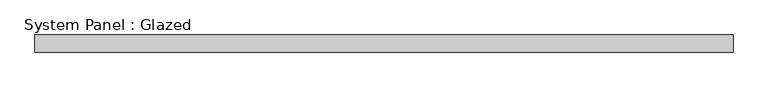
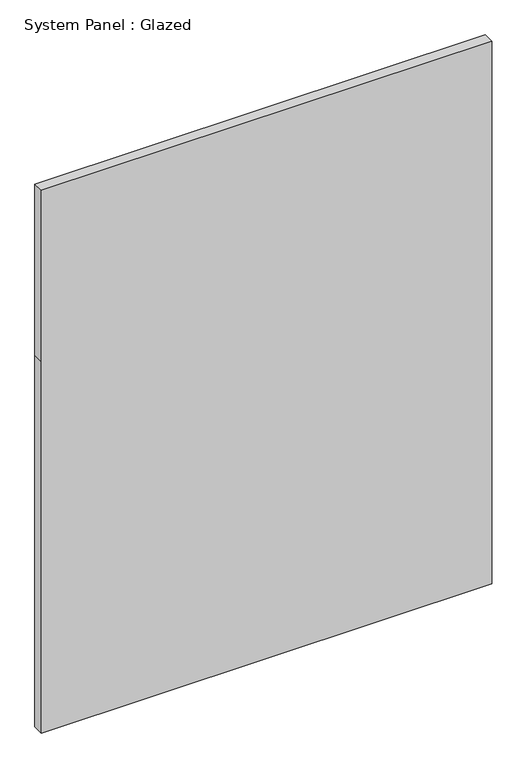
"""IFC4 building model written with IfcOpenShell, lengths in millimetres: plate geometry, System Panel : Glazed."""

from ifc_helpers import new_model, si_unit, frame, origin, place, context, project, spatial, polyline, outline, extrude, source, transform, mapped, element, save


def system_panel_glazed_ed6f96c6(model_context):
    return source(origin(), model_context, "Body", "SweptSolid", [
        extrude(outline(polyline([(0.0, -505.8833333), (0.0, 505.8833333), (882.65, 505.8833333), (1289.05, 505.8833333), (1289.05, -505.8833333), (882.65, -505.8833333), (0.0, -505.8833333)])), frame((0.0, 19.05, 0.0), z_axis=(0.0, 1.0, 0.0), x_axis=(0.0, 0.0, 1.0)), (0.0, 0.0, 1.0), 25.4),
    ])


if __name__ == "__main__":
    model = new_model("IFC4")
    model_context = context("Model", 3, world=origin())
    ifc_project = project(units=[si_unit("LENGTHUNIT", "METRE", prefix="MILLI")], contexts=[model_context])
    site = spatial("IfcSite", under=ifc_project)
    building = spatial("IfcBuilding", under=site)
    placement = place(None, origin())
    system_panel_glazed_shape = system_panel_glazed_ed6f96c6(model_context)
    element("IfcPlate", 1, ObjectType="System Panel : Glazed", at=placement, inside=building, context=model_context, shape_type="MappedRepresentation", body=[
        mapped(system_panel_glazed_shape, transform((0.0, 0.0, 0.0), x_axis=(1.0, 0.0, 0.0), y_axis=(0.0, 1.0, 0.0), z_axis=(0.0, 0.0, 1.0))),
    ])
    save(model, "model.ifc")

# Revit data of these elements
# Type "System Panel : Glazed"
#   Analytic Construction = "1/8 in Pilkington single glazing"
#   Visual Light Transmittance = 0.9
#   Solar Heat Gain Coefficient = 0.86
#   Heat Transfer Coefficient (U) = 1.18115 BTU/(h·ft²·°F)
# Element 1 (IfcPlate, "System Panel : Glazed")
#   Materials on its faces: "Glass, Clear Glazing"
# Materials
#   "Glass, Clear Glazing": class "Glass", colour RGB 245 245 243, transparency 1, Description = "Clear glazing", Cost = 0
